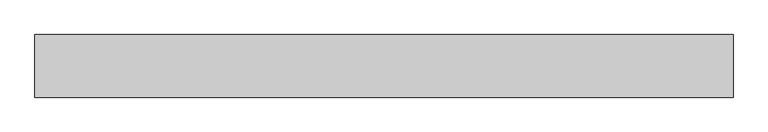
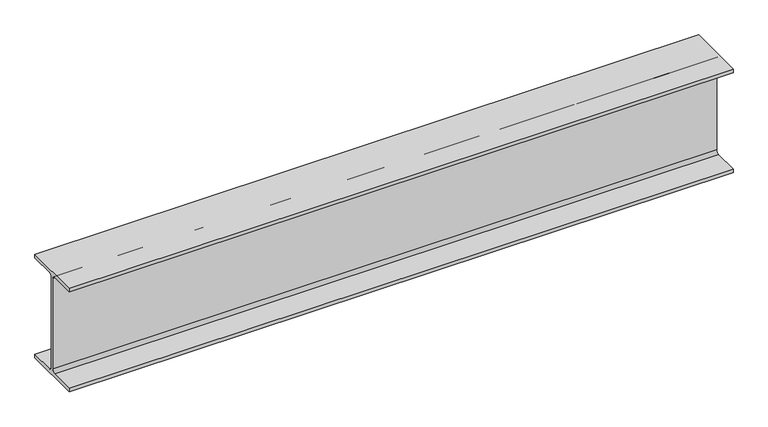
"""IFC4 building model written with IfcOpenShell, lengths in millimetres: beam geometry, Steel Beam_H-KSD3502 : H_SB_ASB_H-194x150x6x9."""

import ifcopenshell
import ifcopenshell.guid

model = None  # the IFC model being written
_history = None  # IfcOwnerHistory: only IFC2X3 demands one
_inside = {}  # id of a spatial element -> (the spatial element, [elements in it])
_under = {}  # id of a project, library or spatial element -> (it, [spatial elements below it])
_declared = {}  # id of a project -> (the project, [libraries it declares])
_typed = {}  # id of a type object -> (the type object, [elements of that type])
_made_of = {}  # id of a material, layer set ... -> (it, [elements and type objects made of it])


def new_model(schema):
    """Start an empty IFC model of exactly this schema.

    Asked for "IFC4X3", IfcOpenShell would pick the latest addendum, in which some entities
    have other attributes; the version numbers below select the first issue.
    IFC2X3 requires an IfcOwnerHistory on every rooted entity: one is made here for all.
    """
    global model, _history
    if schema == "IFC4X3":
        model = ifcopenshell.file(schema_version=(4, 3, 0, 0))
    else:
        model = ifcopenshell.file(schema=schema)
    _inside.clear()
    _under.clear()
    _declared.clear()
    _typed.clear()
    _made_of.clear()
    _history = None
    if model.schema == "IFC2X3":
        org = make("IfcOrganization", Name="unknown")
        user = make(
            "IfcPersonAndOrganization",
            ThePerson=make("IfcPerson", FamilyName="unknown"),
            TheOrganization=org,
        )
        app = make(
            "IfcApplication",
            ApplicationDeveloper=org,
            Version="unknown",
            ApplicationFullName="unknown",
            ApplicationIdentifier="unknown",
        )
        _history = make(
            "IfcOwnerHistory",
            OwningUser=user,
            OwningApplication=app,
            ChangeAction="ADDED",
            CreationDate=0,
        )
    return model


def make(cls, **values):
    """One entity of the class cls with the attributes given. An attribute that is None is left unset."""
    return model.create_entity(
        cls, **{name: value for name, value in values.items() if value is not None}
    )


def rooted(cls, **values):
    """An entity with a GlobalId (a new one), such as an element, a storey or a relation."""
    return make(cls, GlobalId=ifcopenshell.guid.new(), OwnerHistory=_history, **values)


def si_unit(unit_type, name, prefix=None):
    """IfcSIUnit, for example si_unit("LENGTHUNIT", "METRE", prefix="MILLI")."""
    return make("IfcSIUnit", UnitType=unit_type, Prefix=prefix, Name=name)


def assignment(units):
    """IfcUnitAssignment: the units of a project."""
    return None if units is None else make("IfcUnitAssignment", Units=units)


def point(xyz):
    """IfcCartesianPoint."""
    return None if xyz is None else make("IfcCartesianPoint", Coordinates=xyz)


def direction(xyz):
    """IfcDirection."""
    return None if xyz is None else make("IfcDirection", DirectionRatios=xyz)


def frame(location, z_axis=None, x_axis=None):
    """IfcAxis2Placement3D, a coordinate frame: its origin and axes. An axis left out is left unset."""
    return make(
        "IfcAxis2Placement3D",
        Location=point(location),
        Axis=direction(z_axis),
        RefDirection=direction(x_axis),
    )


def frame_2d(location, x_axis=None):
    """IfcAxis2Placement2D, a coordinate frame in the plane: its origin and x axis."""
    return make(
        "IfcAxis2Placement2D", Location=point(location), RefDirection=direction(x_axis)
    )


def origin():
    """The frame at (0, 0, 0) with its axes left unset."""
    return frame((0.0, 0.0, 0.0))


def place(relative_to, where):
    """IfcLocalPlacement: puts the frame where relative to a parent placement (None: the world)."""
    return make(
        "IfcLocalPlacement", PlacementRelTo=relative_to, RelativePlacement=where
    )


def context(
    kind, dimensions, precision=None, world=None, true_north=None, identifier=None
):
    """IfcGeometricRepresentationContext, for example the 3D "Model" context."""
    return make(
        "IfcGeometricRepresentationContext",
        ContextIdentifier=identifier,
        ContextType=kind,
        CoordinateSpaceDimension=dimensions,
        Precision=precision,
        WorldCoordinateSystem=world,
        TrueNorth=true_north,
    )


def project(units=None, contexts=None):
    """IfcProject with its units and contexts."""
    return rooted(
        "IfcProject",
        Name="project",
        RepresentationContexts=contexts,
        UnitsInContext=assignment(units),
    )


def spatial(cls, under=None, at=None, **own):
    """A site, building, storey or space (cls), placed at a placement, below another one or the project."""
    s = rooted(cls, ObjectPlacement=at, **own)
    if under is not None:
        _under.setdefault(under.id(), (under, []))[1].append(s)
    return s


def polyline(points):
    """IfcPolyline through the points."""
    return make("IfcPolyline", Points=[point(p) for p in points])


def circle_curve(where, radius):
    """IfcCircle in the frame where."""
    return make("IfcCircle", Position=where, Radius=radius)


def trimmed(basis, trim1, trim2, sense, master):
    """IfcTrimmedCurve: the piece of a basis curve between two trims."""
    return make(
        "IfcTrimmedCurve",
        BasisCurve=basis,
        Trim1=trim1,
        Trim2=trim2,
        SenseAgreement=sense,
        MasterRepresentation=master,
    )


def segment(curve, same_sense, transition):
    """IfcCompositeCurveSegment."""
    return make(
        "IfcCompositeCurveSegment",
        Transition=transition,
        SameSense=same_sense,
        ParentCurve=curve,
    )


def composite_curve(segments, self_intersect=None):
    """IfcCompositeCurve: segments joined end to end."""
    return make("IfcCompositeCurve", Segments=segments, SelfIntersect=self_intersect)


def outline(outer, holes=None, kind="AREA"):
    """IfcArbitraryClosedProfileDef: a profile drawn as a closed curve; with holes, ...WithVoids."""
    if holes is None:
        return make("IfcArbitraryClosedProfileDef", ProfileType=kind, OuterCurve=outer)
    return make(
        "IfcArbitraryProfileDefWithVoids",
        ProfileType=kind,
        OuterCurve=outer,
        InnerCurves=holes,
    )


def extrude(swept, where, along, depth):
    """IfcExtrudedAreaSolid: the profile swept, set in the frame where, extruded along a direction by depth."""
    return make(
        "IfcExtrudedAreaSolid",
        SweptArea=swept,
        Position=where,
        ExtrudedDirection=direction(along),
        Depth=depth,
    )


def shape(context_of_items, identifier, shape_type, items):
    """IfcShapeRepresentation: the items that make up one representation, for example the "Body"."""
    return make(
        "IfcShapeRepresentation",
        ContextOfItems=context_of_items,
        RepresentationIdentifier=identifier,
        RepresentationType=shape_type,
        Items=items,
    )


def source(mapping_origin, context_of_items, identifier, shape_type, items):
    """IfcRepresentationMap: a shape defined once, which mapped items show again and again."""
    return make(
        "IfcRepresentationMap",
        MappingOrigin=mapping_origin,
        MappedRepresentation=shape(context_of_items, identifier, shape_type, items),
    )


def transform(
    local_origin,
    x_axis=None,
    y_axis=None,
    z_axis=None,
    scale=None,
    scale2=None,
    scale3=None,
    uniform=True,
):
    """IfcCartesianTransformationOperator3D, or its non-uniform kind. x_axis, y_axis, z_axis: its Axis1, 2, 3."""
    if uniform:
        return make(
            "IfcCartesianTransformationOperator3D",
            Axis1=direction(x_axis),
            Axis2=direction(y_axis),
            LocalOrigin=point(local_origin),
            Scale=scale,
            Axis3=direction(z_axis),
        )
    return make(
        "IfcCartesianTransformationOperator3DnonUniform",
        Axis1=direction(x_axis),
        Axis2=direction(y_axis),
        LocalOrigin=point(local_origin),
        Scale=scale,
        Axis3=direction(z_axis),
        Scale2=scale2,
        Scale3=scale3,
    )


def mapped(mapping_source, mapping_target):
    """IfcMappedItem: shows the shape of a source again, moved by a transform."""
    return make(
        "IfcMappedItem", MappingSource=mapping_source, MappingTarget=mapping_target
    )


def made_of(thing, what):
    """Note that an element or type object is made of a material, layer set ...; save() writes the relation."""
    if what is not None:
        _made_of.setdefault(what.id(), (what, []))[1].append(thing)
    return thing


def element(
    cls,
    number,
    at=None,
    inside=None,
    cuts=None,
    type_object=None,
    material=None,
    context=None,
    identifier="Body",
    shape_type=None,
    held_by="IfcProductDefinitionShape",
    body=None,
    shapes=None,
    **own,
):
    """One element of the class cls, such as IfcWall. Its Tag is "e" and its number.

    at: its placement. inside: the storey or other place that contains it. cuts: it is an
    opening in that element (IfcRelVoidsElement). A single representation is given by context,
    identifier, shape_type and body (its items); several are given by shapes. held_by: the class
    of the entity that holds the representations. save() writes the other relations.
    """
    e = rooted(cls, Tag="e%d" % number, ObjectPlacement=at, **own)
    if body is not None:
        shapes = [shape(context, identifier, shape_type, body)]
    if shapes is not None:
        e.Representation = make(held_by, Representations=shapes)
    if inside is not None:
        _inside.setdefault(inside.id(), (inside, []))[1].append(e)
    if cuts is not None:
        rooted(
            "IfcRelVoidsElement", RelatingBuildingElement=cuts, RelatedOpeningElement=e
        )
    if type_object is not None:
        _typed.setdefault(type_object.id(), (type_object, []))[1].append(e)
    return made_of(e, material)


def aggregate(whole, parts):
    """IfcRelAggregates: a whole, such as a stair, and the parts it consists of."""
    return rooted("IfcRelAggregates", RelatingObject=whole, RelatedObjects=parts)


def save(model, path):
    """Write the relations noted so far, then the file.

    IfcRelAggregates (storeys below a building ...), IfcRelContainedInSpatialStructure (elements
    in a storey), IfcRelDefinesByType, IfcRelAssociatesMaterial and IfcRelDeclares: one each for
    every whole, place, type object, material and project.
    """
    for whole, parts in _under.values():
        aggregate(whole, parts)
    for where, things in _inside.values():
        rooted(
            "IfcRelContainedInSpatialStructure",
            RelatedElements=things,
            RelatingStructure=where,
        )
    for kind, things in _typed.values():
        rooted("IfcRelDefinesByType", RelatedObjects=things, RelatingType=kind)
    for what, things in _made_of.values():
        rooted("IfcRelAssociatesMaterial", RelatedObjects=things, RelatingMaterial=what)
    for by, libraries in _declared.values():
        rooted("IfcRelDeclares", RelatingContext=by, RelatedDefinitions=libraries)
    model.write(path)


def beam_885278b6(model_context):
    return source(origin(), model_context, "Body", "SweptSolid", [
        extrude(outline(composite_curve([segment(polyline([(82.5, -141.5), (82.5, -151.7), (-82.5, -151.7), (-82.5, -141.5), (-11.9, -141.5)]), True, "CONTINUOUS"), segment(trimmed(circle_curve(frame_2d((-11.9, -132.6)), 8.9), [point((-11.9, -141.5))], [point((-3.0, -132.6))], True, "CARTESIAN"), True, "CONTINUOUS"), segment(polyline([(-3.0, -132.6), (-3.0, 132.6)]), True, "CONTINUOUS"), segment(trimmed(circle_curve(frame_2d((-11.9, 132.6)), 8.9), [point((-3.0, 132.6))], [point((-11.9, 141.5))], True, "CARTESIAN"), True, "CONTINUOUS"), segment(polyline([(-11.9, 141.5), (-82.5, 141.5), (-82.5, 151.7), (82.5, 151.7), (82.5, 141.5), (11.9, 141.5)]), True, "CONTINUOUS"), segment(trimmed(circle_curve(frame_2d((11.9, 132.6)), 8.9), [point((11.9, 141.5))], [point((3.0, 132.6))], True, "CARTESIAN"), True, "CONTINUOUS"), segment(polyline([(3.0, 132.6), (3.0, -132.6)]), True, "CONTINUOUS"), segment(trimmed(circle_curve(frame_2d((11.9, -132.6)), 8.9), [point((3.0, -132.6))], [point((11.9, -141.5))], True, "CARTESIAN"), True, "CONTINUOUS"), segment(polyline([(11.9, -141.5), (82.5, -141.5)]), True, "CONTINUOUS")], self_intersect=False)), frame((-851.3274068, 0.0, 0.0), z_axis=(1.0, 0.0, 0.0), x_axis=(0.0, 1.0, 0.0)), (0.0, 0.0, 1.0), 1839.6820153),
    ])


if __name__ == "__main__":
    model = new_model("IFC4")
    model_context = context("Model", 3, world=origin())
    ifc_project = project(units=[si_unit("LENGTHUNIT", "METRE", prefix="MILLI")], contexts=[model_context])
    site = spatial("IfcSite", under=ifc_project)
    building = spatial("IfcBuilding", under=site)
    placement = place(None, origin())
    beam_shape = beam_885278b6(model_context)
    element("IfcBeam", 1, ObjectType="Steel Beam_H-KSD3502 : H_SB_ASB_H-194x150x6x9", at=placement, inside=building, context=model_context, shape_type="MappedRepresentation", body=[
        mapped(beam_shape, transform((0.0, 0.0, 0.0), x_axis=(1.0, 0.0, 0.0), y_axis=(0.0, 1.0, 0.0), z_axis=(0.0, 0.0, 1.0))),
    ])
    save(model, "model.ifc")

# Revit data of these elements
# Type "Steel Beam_H-KSD3502 : H_SB_ASB_H-194x150x6x9"
#   Width = 15.0 cm
#   Web Thickness = 0.6 cm
#   Web Fillet = 1.3 cm
#   Warping Constant = 43316.0 cm⁶
#   Torsional Moment of Inertia = 8.622 cm⁴
#   Torsional Modulus = 1.0 cm³
#   Section Area = 39.01 cm²
#   Plastic Modulus weak axis = 104.0 cm³
#   Plastic Modulus strong axis = 309.0 cm³
#   Perimeter = 0.95 m²/m
#   Nominal Weight = 30.60 kgf/m
#   Moment of Inertia weak axis = 507.00 cm⁴
#   Moment of Inertia strong axis = 2690.00 cm⁴
#   Height = 19.4 cm
#   Flange Thickness = 0.9 cm
#   Elastic Modulus weak axis = 67.6 cm³
#   Elastic Modulus strong axis = 277.0 cm³
#   Centroid Vertical = 9.7 cm
#   Centroid Horizontal = 7.5 cm
#   Length [instance default] = 1.5240 m
#   Structural Material [instance default] = Steel, 45-345
#   Assembly Code = ""
# Element 1 (IfcBeam, "Steel Beam_H-KSD3502 : H_SB_ASB_H-194x150x6x9")
#   Structural Material = none
# Materials
#   "Steel, 45-345": class "Metal", colour RGB 189 187 185, transparency 0, Description = "Steel 345 MPa", Cost = 0
